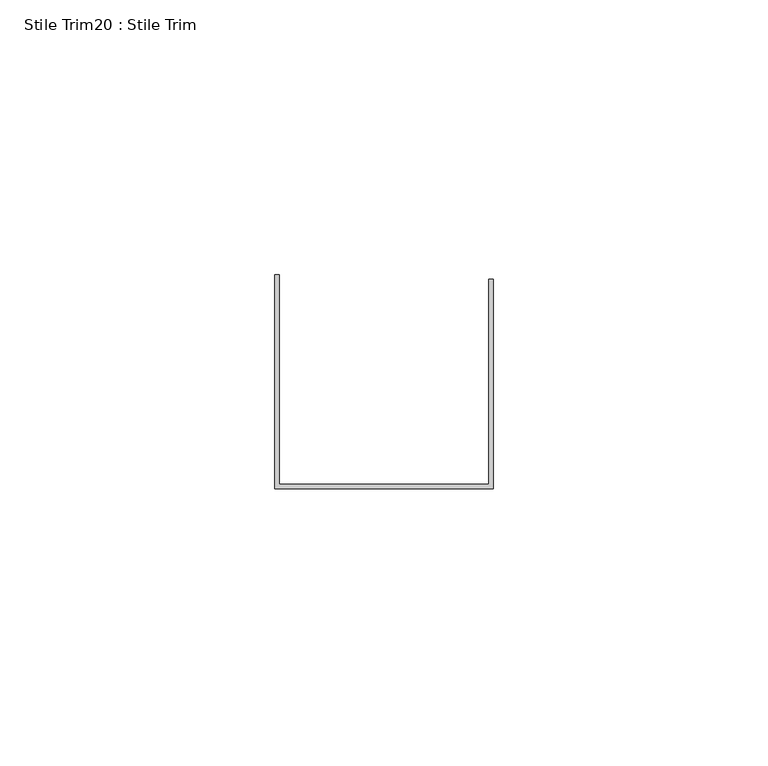
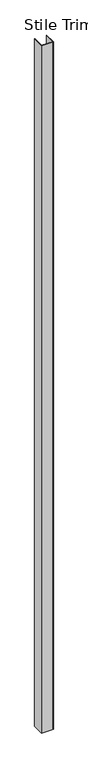
"""IFC4 building model written with IfcOpenShell, lengths in millimetres: proxy geometry, Stile Trim20 : Stile Trim."""

from ifc_helpers import new_model, si_unit, frame, origin, place, context, project, spatial, polyline, outline, extrude, source, transform, mapped, element, save


def stile_trim20_stile_trim_7538b4aa(model_context):
    return source(origin(), model_context, "Body", "SweptSolid", [
        extrude(outline(polyline([(587327.0060739, -531776.5287841), (587327.0060739, -531737.6413841), (587327.7934739, -531737.6413841), (587327.7934739, -531775.7413841), (587365.8934739, -531775.7413841), (587365.8934739, -531738.4287841), (587366.6808739, -531738.4287841), (587366.6808739, -531776.5287841), (587327.0060739, -531776.5287841)])), frame((0.0, 0.0, 11.90625), z_axis=(0.0, 0.0, 1.0), x_axis=(1.0, 0.0, 0.0)), (0.0, 0.0, 1.0), 2426.49375),
    ])


if __name__ == "__main__":
    model = new_model("IFC4")
    model_context = context("Model", 3, world=origin())
    ifc_project = project(units=[si_unit("LENGTHUNIT", "METRE", prefix="MILLI")], contexts=[model_context])
    site = spatial("IfcSite", under=ifc_project)
    building = spatial("IfcBuilding", under=site)
    placement = place(None, origin())
    stile_trim20_stile_trim_shape = stile_trim20_stile_trim_7538b4aa(model_context)
    element("IfcBuildingElementProxy", 1, Name="Stile Trim20 : Stile Trim", ObjectType="Stile Trim20 : Stile Trim", at=placement, inside=building, context=model_context, shape_type="MappedRepresentation", body=[
        mapped(stile_trim20_stile_trim_shape, transform((0.0, 0.0, 0.0), x_axis=(1.0, 0.0, 0.0), y_axis=(0.0, 1.0, 0.0), z_axis=(0.0, 0.0, 1.0))),
    ])
    save(model, "model.ifc")

# Revit data of these elements
# Element 1 (IfcBuildingElementProxy, "Stile Trim20 : Stile Trim")
#   Materials on its faces: "EDGE TRIM BY MTL PANEL MFR."
# Materials
#   "EDGE TRIM BY MTL PANEL MFR.": class "Generic", colour RGB 239 242 240, transparency 0, Cost = 0
